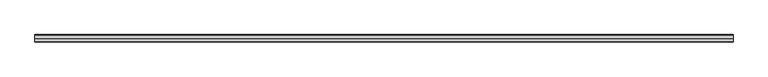
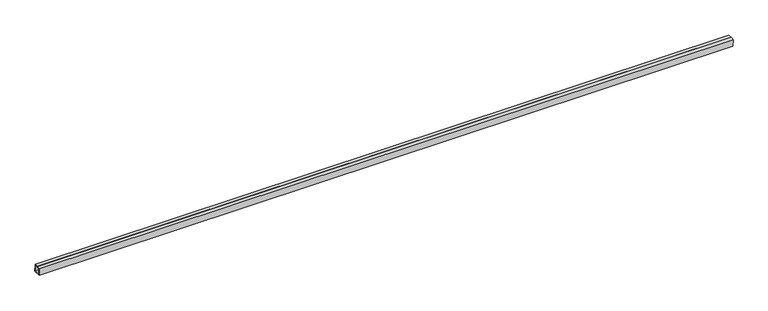
"""IFC4 building model written with IfcOpenShell, lengths in millimetres: proxy geometry, Inner panel:Inner panel:1:Inner panel:1 : Inner panel:Inner panel:300324:2:Inner panel:1:Inner panel:1 : Inner panel:Inner panel:300324:2 : Inner panel:Inner panel:1:Inner panel:1 : Inner panel:Inner panel:300324:300043:14 : Inner panel:Inner panel:1:Inner panel:1 : Inner panel:Inner panel:300324:2:Inner panel:1:Inner panel:1 : Inner panel:Inner panel:300324:2 : Inner panel:Inner panel:1:Inner panel:1 : Inner panel:Inner panel:300324:300043:308120."""

from ifc_helpers import new_model, si_unit, frame, origin, place, context, project, spatial, polyline, outline, extrude, source, transform, mapped, element, save


def generic_models_1421dc05(model_context):
    return source(origin(), model_context, "Body", "SweptSolid", [
        extrude(outline(polyline([(-568274.9584236, 8800.0160778), (-568256.7180004, 8800.7760955), (-568255.1318767, 8762.7091254), (-568293.1988468, 8761.1230016), (-568294.7849705, 8799.1899717), (-568276.5445474, 8799.9499893), (-568276.4454146, 8797.5708037), (-568292.3066522, 8796.9099188), (-568290.9187939, 8763.60132), (-568257.6101951, 8764.9891783), (-568258.9980533, 8798.2977771), (-568274.8592909, 8797.6368922), (-568274.9584236, 8800.0160778)])), frame((593141.1867242, 0.0, 0.0), z_axis=(1.0, 0.0, 0.0), x_axis=(0.0, 1.0, 0.0)), (0.0, 0.0, 1.0), 3657.6),
    ])


if __name__ == "__main__":
    model = new_model("IFC4")
    model_context = context("Model", 3, world=origin())
    ifc_project = project(units=[si_unit("LENGTHUNIT", "METRE", prefix="MILLI")], contexts=[model_context])
    site = spatial("IfcSite", under=ifc_project)
    building = spatial("IfcBuilding", under=site)
    placement = place(None, origin())
    generic_models_shape = generic_models_1421dc05(model_context)
    element("IfcBuildingElementProxy", 1, Name="Inner panel:Inner panel:1:Inner panel:1 : Inner panel:Inner panel:300324:2:Inner panel:1:Inner panel:1 : Inner panel:Inner panel:300324:2 : Inner panel:Inner panel:1:Inner panel:1 : Inner panel:Inner panel:300324:300043:14 : Inner panel:Inner panel:1:Inner panel:1 : Inner panel:Inner panel:300324:2:Inner panel:1:Inner panel:1 : Inner panel:Inner panel:300324:2 : Inner panel:Inner panel:1:Inner panel:1 : Inner panel:Inner panel:300324:300043:308120", ObjectType="Inner panel:Inner panel:1:Inner panel:1 : Inner panel:Inner panel:300324:2:Inner panel:1:Inner panel:1 : Inner panel:Inner panel:300324:2 : Inner panel:Inner panel:1:Inner panel:1 : Inner panel:Inner panel:300324:300043:14 : Inner panel:Inner panel:1:Inner panel:1 : Inner panel:Inner panel:300324:2:Inner panel:1:Inner panel:1 : Inner panel:Inner panel:300324:2 : Inner panel:Inner panel:1:Inner panel:1 : Inner panel:Inner panel:300324:300043:308120", at=placement, inside=building, context=model_context, shape_type="MappedRepresentation", body=[
        mapped(generic_models_shape, transform((0.0, 0.0, 0.0), x_axis=(1.0, 0.0, 0.0), y_axis=(0.0, 1.0, 0.0), z_axis=(0.0, 0.0, 1.0))),
    ])
    save(model, "model.ifc")

# Revit data of these elements
# Type "Inner panel:Inner panel:1:Inner panel:1 : Inner panel:Inner panel:300324:2:Inner panel:1:Inner panel:1 : Inner panel:Inner panel:300324:2 : Inner panel:Inner panel:1:Inner panel:1 : Inner panel:Inner panel:300324:300043:14 : Inner panel:Inner panel:1:Inner panel:1 : Inner panel:Inner panel:300324:2:Inner panel:1:Inner panel:1 : Inner panel:Inner panel:300324:2 : Inner panel:Inner panel:1:Inner panel:1 : Inner panel:Inner panel:300324:300043:308120"
#   NameOverride = "Inner panel:Inner panel:1:Inner panel:1 : Inner panel:Inner panel:300324:2:Inner panel:1:Inner panel:1 : Inner panel:Inner panel:300324:2 : Inner panel:Inner panel:1:Inner panel:1 : Inner panel:Inner panel:300324:300043:308120"
#   ObjectTypeOverride = "Inner panel:1:Inner panel:1 : Inner panel:Inner panel:300324:2 : Inner panel:Inner panel:1:Inner panel:1 : Inner panel:Inner panel:300324:300043"
#   Reference = "Inner panel"
#   Tag = "308120"
# Element 1 (IfcBuildingElementProxy, "Inner panel:Inner panel:1:Inner panel:1 : Inner panel:Inner panel:300324:2:Inner panel:1:Inner panel:1 : Inner panel:Inner panel:300324:2 : Inner panel:Inner panel:1:Inner panel:1 : Inner panel:Inner panel:300324:300043:14 : Inner panel:Inner panel:1:Inner panel:1 : Inner panel:Inner panel:300324:2:Inner panel:1:Inner panel:1 : Inner panel:Inner panel:300324:2 : Inner panel:Inner panel:1:Inner panel:1 : Inner panel:Inner panel:300324:300043:308120")
#   Materials on its faces: "1 1/2\" X 1 1/2\" SPLIT-SEAM SQUARE TUBING (~24\" CANTILEVER FROM C.L. OF GLULAM)"
# Materials
#   "1 1/2\" X 1 1/2\" SPLIT-SEAM SQUARE TUBING (~24\" CANTILEVER FROM C.L. OF GLULAM)": class "Unassigned", colour RGB 202 201 200, transparency 0, Cost = 0
